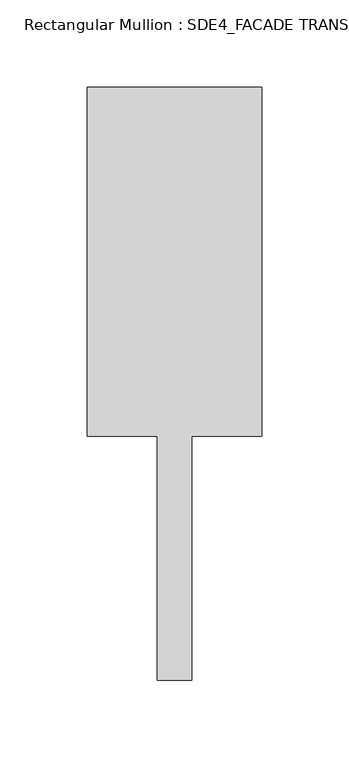
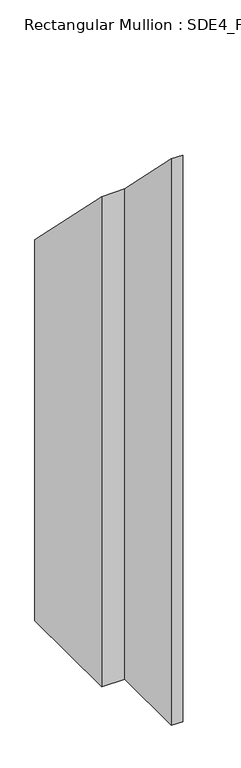
"""IFC4 building model written with IfcOpenShell, lengths in millimetres: member geometry, Rectangular Mullion : SDE4_FACADE TRANSOM TYPE 1."""

from ifc_helpers import new_model, si_unit, origin, place, context, project, spatial, faceted_brep, source, transform, mapped, element, save


def rectangular_mullion_sde4_facade_transom_type_1_71476849(model_context):
    return source(origin(), model_context, "Body", "Brep", [
        faceted_brep([(50.0, 132.5, -830.5990258), (50.0, -67.5, -830.5990258), (10.0, -67.5, -830.5990258), (10.0, -207.5, -830.5990258), (-10.0, -207.5, -830.5990258), (-10.0, -67.5, -830.5990258), (-50.0, -67.5, -830.5990258), (-50.0, 132.5, -830.5990258), (-50.0, 132.5, -132.5), (50.0, 132.5, -132.5), (-50.0, -67.5, 67.5), (-10.0, -67.5, 67.5), (-10.0, -207.5, 207.5), (10.0, -207.5, 207.5), (10.0, -67.5, 67.5), (50.0, -67.5, 67.5)], [[[0, 1, 2, 3, 4, 5, 6, 7]], [[8, 9, 0, 7]], [[10, 8, 7, 6]], [[11, 10, 6, 5]], [[12, 11, 5, 4]], [[13, 12, 4, 3]], [[14, 13, 3, 2]], [[15, 14, 2, 1]], [[9, 15, 1, 0]], [[9, 8, 10, 11, 12, 13, 14, 15]]]),
    ])


if __name__ == "__main__":
    model = new_model("IFC4")
    model_context = context("Model", 3, world=origin())
    ifc_project = project(units=[si_unit("LENGTHUNIT", "METRE", prefix="MILLI")], contexts=[model_context])
    site = spatial("IfcSite", under=ifc_project)
    building = spatial("IfcBuilding", under=site)
    placement = place(None, origin())
    rectangular_mullion_sde4_facade_transom_type_1_shape = rectangular_mullion_sde4_facade_transom_type_1_71476849(model_context)
    element("IfcMember", 1, ObjectType="Rectangular Mullion : SDE4_FACADE TRANSOM TYPE 1", at=placement, inside=building, context=model_context, shape_type="MappedRepresentation", body=[
        mapped(rectangular_mullion_sde4_facade_transom_type_1_shape, transform((0.0, 0.0, 0.0), x_axis=(1.0, 0.0, 0.0), y_axis=(0.0, 1.0, 0.0), z_axis=(0.0, 0.0, 1.0))),
    ])
    save(model, "model.ifc")

# Revit data of these elements
# Type "Rectangular Mullion : SDE4_FACADE TRANSOM TYPE 1"
#   built-in parameter 1007322 = 1.11549 (stored number, unit not read)
#   built-in parameter 1007321 = 0.164042 (stored number, unit not read)
#   built-in parameter 1007320 = 0.164042 (stored number, unit not read)
